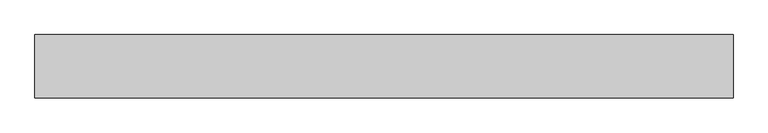
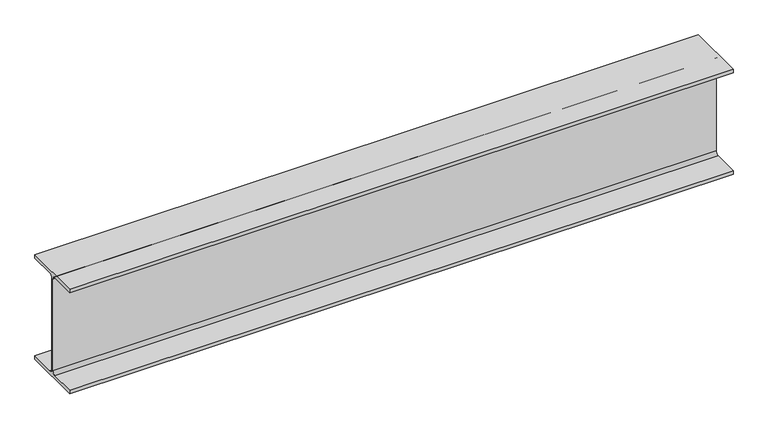
"""IFC4 building model written with IfcOpenShell, lengths in millimetres: beam geometry, Old_Steel Beam_H-KSD3502 : H_SB_ASB_H-194×150x6x9."""

from ifc_helpers import new_model, si_unit, point, frame, frame_2d, origin, place, context, project, spatial, polyline, circle_curve, trimmed, segment, composite_curve, outline, extrude, source, transform, mapped, element, save


def beam_7401761e(model_context):
    return source(origin(), model_context, "Body", "SweptSolid", [
        extrude(outline(composite_curve([segment(polyline([(-82.5, -141.5), (-11.9, -141.5)]), True, "CONTINUOUS"), segment(trimmed(circle_curve(frame_2d((-11.9, -132.6)), 8.9), [point((-11.9, -141.5))], [point((-3.0, -132.6))], True, "CARTESIAN"), True, "CONTINUOUS"), segment(polyline([(-3.0, -132.6), (-3.0, 132.6)]), True, "CONTINUOUS"), segment(trimmed(circle_curve(frame_2d((-11.9, 132.6)), 8.9), [point((-3.0, 132.6))], [point((-11.9, 141.5))], True, "CARTESIAN"), True, "CONTINUOUS"), segment(polyline([(-11.9, 141.5), (-82.5, 141.5), (-82.5, 151.7), (82.5, 151.7), (82.5, 141.5), (11.9, 141.5)]), True, "CONTINUOUS"), segment(trimmed(circle_curve(frame_2d((11.9, 132.6)), 8.9), [point((11.9, 141.5))], [point((3.0, 132.6))], True, "CARTESIAN"), True, "CONTINUOUS"), segment(polyline([(3.0, 132.6), (3.0, -132.6)]), True, "CONTINUOUS"), segment(trimmed(circle_curve(frame_2d((11.9, -132.6)), 8.9), [point((3.0, -132.6))], [point((11.9, -141.5))], True, "CARTESIAN"), True, "CONTINUOUS"), segment(polyline([(11.9, -141.5), (82.5, -141.5), (82.5, -151.7), (-82.5, -151.7), (-82.5, -141.5)]), True, "CONTINUOUS")], self_intersect=False)), frame((-908.9645727, 0.0, 0.0), z_axis=(1.0, 0.0, 0.0), x_axis=(0.0, 1.0, 0.0)), (0.0, 0.0, 1.0), 1817.9291455),
    ])


if __name__ == "__main__":
    model = new_model("IFC4")
    model_context = context("Model", 3, world=origin())
    ifc_project = project(units=[si_unit("LENGTHUNIT", "METRE", prefix="MILLI")], contexts=[model_context])
    site = spatial("IfcSite", under=ifc_project)
    building = spatial("IfcBuilding", under=site)
    placement = place(None, origin())
    beam_shape = beam_7401761e(model_context)
    element("IfcBeam", 1, ObjectType="Old_Steel Beam_H-KSD3502 : H_SB_ASB_H-194×150x6x9", at=placement, inside=building, context=model_context, shape_type="MappedRepresentation", body=[
        mapped(beam_shape, transform((0.0, 0.0, 0.0), x_axis=(1.0, 0.0, 0.0), y_axis=(0.0, 1.0, 0.0), z_axis=(0.0, 0.0, 1.0))),
    ])
    save(model, "model.ifc")

# Revit data of these elements
# Type "Old_Steel Beam_H-KSD3502 : H_SB_ASB_H-194×150x6x9"
#   Width = 15.0 cm
#   Web Thickness = 0.6 cm
#   Web Fillet = 1.3 cm
#   Warping Constant = 43316.0 cm⁶
#   Torsional Moment of Inertia = 8.622 cm⁴
#   Torsional Modulus = 1.0 cm³
#   Section Area = 39.01 cm²
#   Plastic Modulus weak axis = 104.0 cm³
#   Plastic Modulus strong axis = 309.0 cm³
#   Perimeter = 0.95 m²/m
#   Nominal Weight = 30.60 kgf/m
#   Moment of Inertia weak axis = 507.00 cm⁴
#   Moment of Inertia strong axis = 2690.00 cm⁴
#   Height = 19.4 cm
#   Flange Thickness = 0.9 cm
#   Elastic Modulus weak axis = 67.6 cm³
#   Elastic Modulus strong axis = 277.0 cm³
#   Centroid Vertical = 9.7 cm
#   Centroid Horizontal = 7.5 cm
#   Length [instance default] = 1.5240 m
#   Structural Material [instance default] = Steel, 45-345
#   Assembly Code = ""
# Element 1 (IfcBeam, "Old_Steel Beam_H-KSD3502 : H_SB_ASB_H-194×150x6x9")
#   Structural Material = none
# Materials
#   "Steel, 45-345": class "Metal", colour RGB 189 187 185, transparency 0, Description = "Steel 345 MPa", Cost = 0
